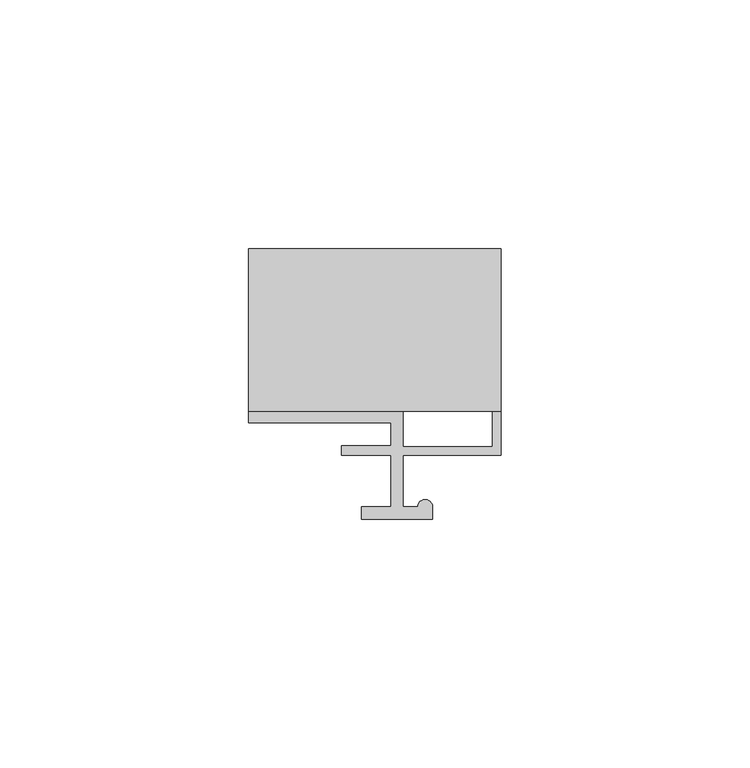
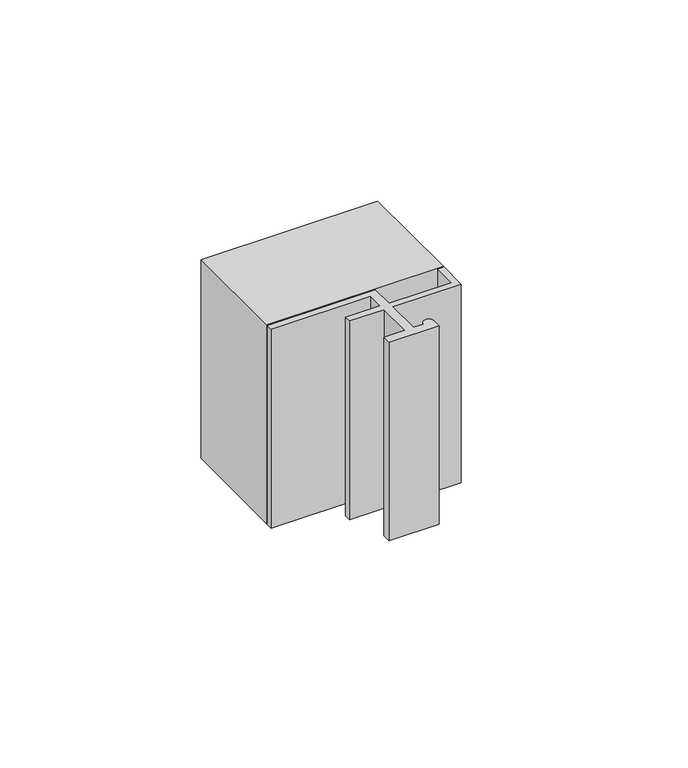
"""IFC4 building model written with IfcOpenShell, lengths in millimetres: proxy geometry, Generic Models 9:Generic Models 5:348123:Generic Models 5:348123 : Generic Models 9:Generic Models 5:348123:4 : Generic Models 9:Generic Models 5:348123:Generic Models 5:348123 : Generic Models 9:Generic Models 5:348123:301771."""

from ifc_helpers import new_model, si_unit, point, frame, frame_2d, origin, place, context, project, spatial, polyline, circle_curve, trimmed, segment, composite_curve, outline, extrude, source, transform, mapped, element, save


def generic_models_a4aad022(model_context):
    return source(origin(), model_context, "Body", "SweptSolid", [
        extrude(outline(polyline([(593279.408438, -568186.6413841), (593330.208438, -568186.6413841), (593330.208438, -568219.2983921), (593279.408438, -568219.2983921), (593279.408438, -568186.6413841)])), frame((0.0, 0.0, 7316.010103), z_axis=(0.0, 0.0, 1.0), x_axis=(1.0, 0.0, 0.0)), (0.0, 0.0, 1.0), 60.325),
        extrude(outline(composite_curve([segment(polyline([(593310.4802827, -568228.176062), (593310.4802827, -568238.5333435), (593313.439506, -568238.5333435)]), True, "CONTINUOUS"), segment(trimmed(circle_curve(frame_2d((593314.9191176, -568238.5333435)), 1.4796117), [point((593313.439506, -568238.5333435))], [point((593316.3987293, -568238.5333435))], False, "CARTESIAN"), True, "CONTINUOUS"), segment(polyline([(593316.3987293, -568238.5333435), (593316.3987293, -568240.9993629), (593302.0958166, -568240.9993629), (593302.0958166, -568238.5333435), (593308.0142632, -568238.5333435), (593308.0142632, -568228.176062), (593298.1501856, -568228.176062), (593298.1501856, -568226.2032464), (593308.0142632, -568226.2032464), (593308.0142632, -568221.5671299), (593279.408438, -568221.5671299), (593279.408438, -568219.2983921), (593310.4802827, -568219.2983921), (593310.4802827, -568226.400528), (593328.432904, -568226.400528), (593328.432904, -568219.2983921), (593330.208438, -568219.2983921), (593330.208438, -568228.176062), (593310.4802827, -568228.176062)]), True, "CONTINUOUS")], self_intersect=False)), frame((0.0, 0.0, 7316.010103), z_axis=(0.0, 0.0, 1.0), x_axis=(1.0, 0.0, 0.0)), (0.0, 0.0, 1.0), 60.325),
    ])


if __name__ == "__main__":
    model = new_model("IFC4")
    model_context = context("Model", 3, world=origin())
    ifc_project = project(units=[si_unit("LENGTHUNIT", "METRE", prefix="MILLI")], contexts=[model_context])
    site = spatial("IfcSite", under=ifc_project)
    building = spatial("IfcBuilding", under=site)
    placement = place(None, origin())
    generic_models_shape = generic_models_a4aad022(model_context)
    element("IfcBuildingElementProxy", 1, Name="Generic Models 9:Generic Models 5:348123:Generic Models 5:348123 : Generic Models 9:Generic Models 5:348123:4 : Generic Models 9:Generic Models 5:348123:Generic Models 5:348123 : Generic Models 9:Generic Models 5:348123:301771", ObjectType="Generic Models 9:Generic Models 5:348123:Generic Models 5:348123 : Generic Models 9:Generic Models 5:348123:4 : Generic Models 9:Generic Models 5:348123:Generic Models 5:348123 : Generic Models 9:Generic Models 5:348123:301771", at=placement, inside=building, context=model_context, shape_type="MappedRepresentation", body=[
        mapped(generic_models_shape, transform((0.0, 0.0, 0.0), x_axis=(1.0, 0.0, 0.0), y_axis=(0.0, 1.0, 0.0), z_axis=(0.0, 0.0, 1.0))),
    ])
    save(model, "model.ifc")

# Revit data of these elements
# Type "Generic Models 9:Generic Models 5:348123:Generic Models 5:348123 : Generic Models 9:Generic Models 5:348123:4 : Generic Models 9:Generic Models 5:348123:Generic Models 5:348123 : Generic Models 9:Generic Models 5:348123:301771"
#   NameOverride = "Generic Models 9:Generic Models 5:348123:Generic Models 5:348123 : Generic Models 9:Generic Models 5:348123:301771"
#   ObjectTypeOverride = "Generic Models 5:348123 : Generic Models 9:Generic Models 5:348123"
#   Reference = "Generic Models 5"
#   Tag = "301771"
# Element 1 (IfcBuildingElementProxy, "Generic Models 9:Generic Models 5:348123:Generic Models 5:348123 : Generic Models 9:Generic Models 5:348123:4 : Generic Models 9:Generic Models 5:348123:Generic Models 5:348123 : Generic Models 9:Generic Models 5:348123:301771")
#   Materials on its faces: "GALVANIZED STEEL CLIP AT EVERY SEAM IN POLYCARBONATE"
# Materials
#   "GALVANIZED STEEL CLIP AT EVERY SEAM IN POLYCARBONATE": class "Unassigned", colour RGB 120 120 120, transparency 0, Cost = 0
